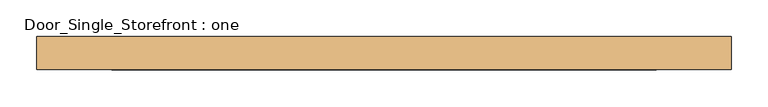
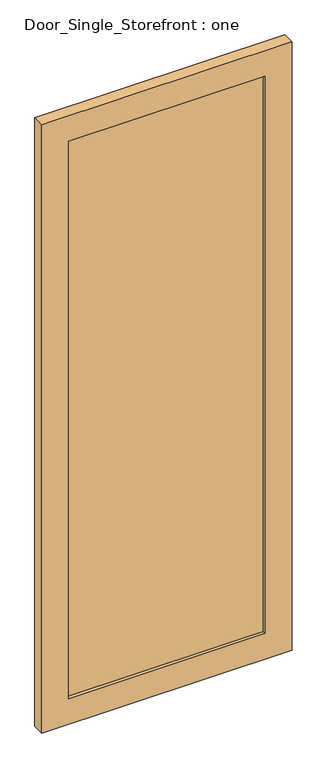
"""IFC4 building model written with IfcOpenShell, lengths in millimetres: door geometry, Door_Single_Storefront : one."""

from ifc_helpers import new_model, si_unit, frame, origin, place, context, project, spatial, polyline, outline, extrude, source, transform, mapped, element, save


def door_single_storefront_one_5048e902(model_context):
    return source(origin(), model_context, "Body", "SweptSolid", [
        extrude(outline(polyline([(368.3, 19.05), (-368.3, 19.05), (-368.3, 38.1), (368.3, 38.1), (368.3, 19.05)])), frame((0.0, 0.0, 101.6), z_axis=(0.0, 0.0, 1.0), x_axis=(1.0, 0.0, 0.0)), (0.0, 0.0, 1.0), 2209.8),
        extrude(outline(polyline([(2413.0, -469.9), (0.0, -469.9), (0.0, 469.9), (2413.0, 469.9), (2413.0, -469.9)]), holes=[polyline([(101.6, 368.3), (101.6, -368.3), (2311.4, -368.3), (2311.4, 368.3), (101.6, 368.3)])]), frame((0.0, 6.35, 0.0), z_axis=(0.0, 1.0, 0.0), x_axis=(0.0, 0.0, 1.0)), (0.0, 0.0, 1.0), 44.45),
    ])


if __name__ == "__main__":
    model = new_model("IFC4")
    model_context = context("Model", 3, world=origin())
    ifc_project = project(units=[si_unit("LENGTHUNIT", "METRE", prefix="MILLI")], contexts=[model_context])
    site = spatial("IfcSite", under=ifc_project)
    building = spatial("IfcBuilding", under=site)
    placement = place(None, origin())
    door_single_storefront_one_shape = door_single_storefront_one_5048e902(model_context)
    element("IfcDoor", 1, ObjectType="Door_Single_Storefront : one", at=placement, inside=building, context=model_context, shape_type="MappedRepresentation", body=[
        mapped(door_single_storefront_one_shape, transform((0.0, 0.0, 0.0), x_axis=(1.0, 0.0, 0.0), y_axis=(0.0, 1.0, 0.0), z_axis=(0.0, 0.0, 1.0))),
    ])
    save(model, "model.ifc")

# Revit data of these elements
# Type "Door_Single_Storefront : one"
#   Type Mark = "27"
#   Analytic Construction = "<None>"
#   Stile_Width = 0' - 4"
#   Door_Thickness = 0' - 1 3/4"
#   Door_Offset = 0' - 2"
#   Glass_Material = Glass
#   Frame_Material = Aluminum
#   Function = (empty or 0)
# Element 1 (IfcDoor, "Door_Single_Storefront : one")
#   Materials on its faces: "Aluminum", "Glass"
# Materials
#   "Glass": class "Glass", colour RGB 0 128 192, transparency 0.75, Description = "Soda Lime Glass", Cost = 0
#   "Aluminum": class "Metal", colour RGB 247 247 247, transparency 0, Description = "Aluminum 6061", Cost = 0
